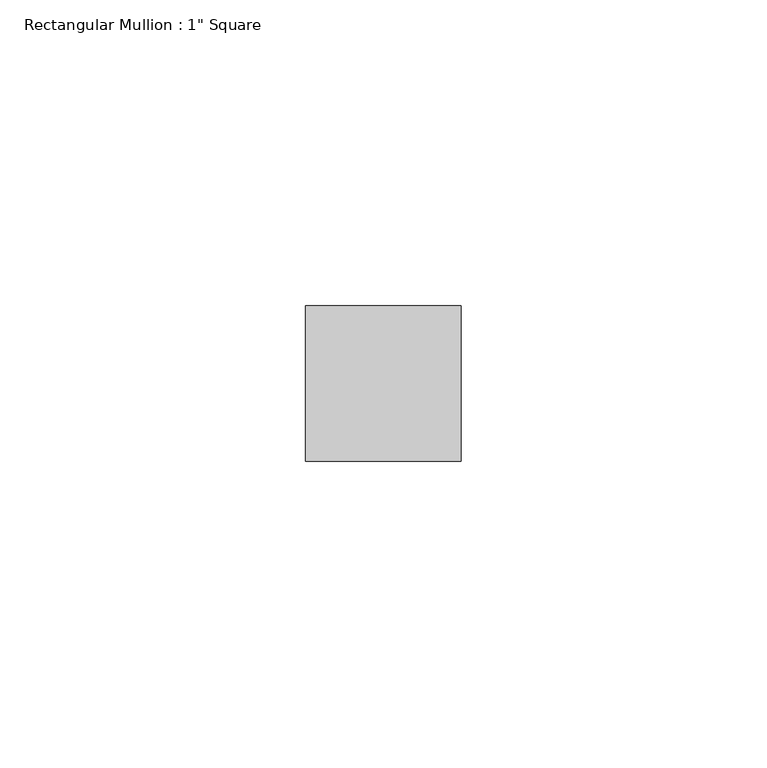
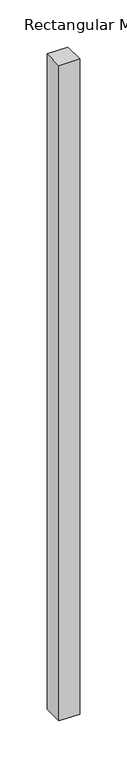
"""IFC4 building model written with IfcOpenShell, lengths in millimetres: member geometry."""

from ifc_helpers import new_model, si_unit, frame, origin, place, context, project, spatial, polyline, outline, extrude, source, transform, mapped, element, save


def member_33e43737(model_context):
    return source(origin(), model_context, "Body", "SweptSolid", [
        extrude(outline(polyline([(0.0, 12.7), (0.0, -12.7), (-25.4, -12.7), (-25.4, 12.7), (0.0, 12.7)])), frame((0.0, 0.0, -850.8999997), z_axis=(0.0, 0.0, 1.0), x_axis=(1.0, 0.0, 0.0)), (0.0, 0.0, 1.0), 850.8999997),
    ])


if __name__ == "__main__":
    model = new_model("IFC4")
    model_context = context("Model", 3, world=origin())
    ifc_project = project(units=[si_unit("LENGTHUNIT", "METRE", prefix="MILLI")], contexts=[model_context])
    site = spatial("IfcSite", under=ifc_project)
    building = spatial("IfcBuilding", under=site)
    placement = place(None, origin())
    member_shape = member_33e43737(model_context)
    element("IfcMember", 1, ObjectType="Rectangular Mullion : 1\" Square", at=placement, inside=building, context=model_context, shape_type="MappedRepresentation", body=[
        mapped(member_shape, transform((0.0, 0.0, 0.0), x_axis=(1.0, 0.0, 0.0), y_axis=(0.0, 1.0, 0.0), z_axis=(0.0, 0.0, 1.0))),
    ])
    save(model, "model.ifc")

# Revit data of these elements
# Type "Rectangular Mullion : 1\" Square"
#   built-in parameter 1007304 = 0.0833333 (stored number, unit not read)
#   built-in parameter 1007301 = 0.0416667 (stored number, unit not read)
#   built-in parameter 1007300 = 0.0416667 (stored number, unit not read)
# Element 1 (IfcMember, "Rectangular Mullion : 1\" Square")
#   Materials on its faces: "Metal - Aluminum"
# Materials
#   "Metal - Aluminum": class "Metal", colour RGB 247 247 247, transparency 0
